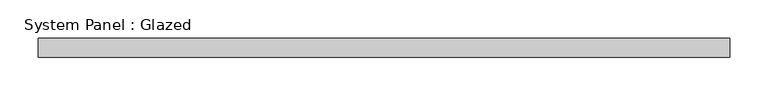
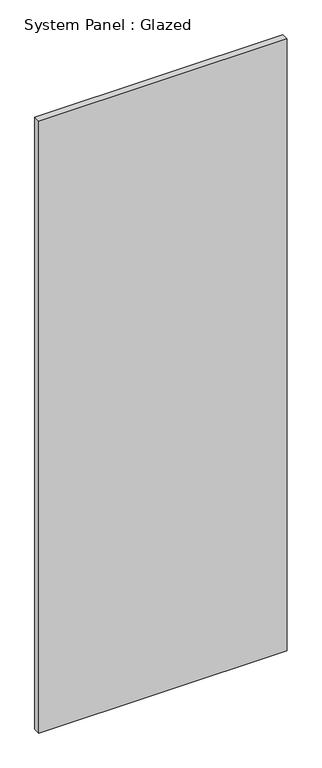
"""IFC4 building model written with IfcOpenShell, lengths in millimetres: plate geometry, System Panel : Glazed."""

from ifc_helpers import new_model, si_unit, origin, origin_with_axes, place, context, project, spatial, polyline, outline, extrude, source, transform, mapped, element, save


def system_panel_glazed_49c13c4b(model_context):
    return source(origin(), model_context, "Body", "SweptSolid", [
        extrude(outline(polyline([(453.5714285, -12.7), (-453.5714285, -12.7), (-453.5714285, 12.7), (453.5714285, 12.7), (453.5714285, -12.7)])), origin_with_axes(), (0.0, 0.0, 1.0), 2362.2),
    ])


if __name__ == "__main__":
    model = new_model("IFC4")
    model_context = context("Model", 3, world=origin())
    ifc_project = project(units=[si_unit("LENGTHUNIT", "METRE", prefix="MILLI")], contexts=[model_context])
    site = spatial("IfcSite", under=ifc_project)
    building = spatial("IfcBuilding", under=site)
    placement = place(None, origin())
    system_panel_glazed_shape = system_panel_glazed_49c13c4b(model_context)
    element("IfcPlate", 1, ObjectType="System Panel : Glazed", at=placement, inside=building, context=model_context, shape_type="MappedRepresentation", body=[
        mapped(system_panel_glazed_shape, transform((0.0, 0.0, 0.0), x_axis=(1.0, 0.0, 0.0), y_axis=(0.0, 1.0, 0.0), z_axis=(0.0, 0.0, 1.0))),
    ])
    save(model, "model.ifc")

# Revit data of these elements
# Element 1 (IfcPlate, "System Panel : Glazed")
#   Materials on its faces: "Glass"
# Materials
#   "Glass": class "Glass", colour RGB 218 227 224, transparency 0.85, Description = "Soda Lime Glass", Cost = 0
